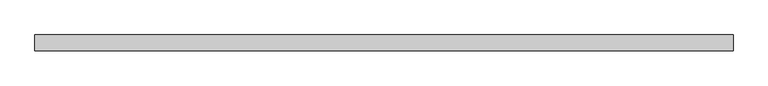
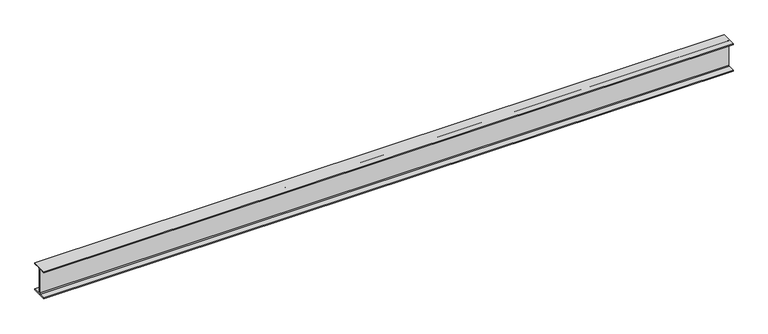
"""IFC4 building model written with IfcOpenShell, lengths in millimetres: beam geometry, Old_Steel Beam_H-KSD3502 : H_SB_ASB_H-390×300x10x16."""

import ifcopenshell
import ifcopenshell.guid

model = None  # the IFC model being written
_history = None  # IfcOwnerHistory: only IFC2X3 demands one
_inside = {}  # id of a spatial element -> (the spatial element, [elements in it])
_under = {}  # id of a project, library or spatial element -> (it, [spatial elements below it])
_declared = {}  # id of a project -> (the project, [libraries it declares])
_typed = {}  # id of a type object -> (the type object, [elements of that type])
_made_of = {}  # id of a material, layer set ... -> (it, [elements and type objects made of it])


def new_model(schema):
    """Start an empty IFC model of exactly this schema.

    Asked for "IFC4X3", IfcOpenShell would pick the latest addendum, in which some entities
    have other attributes; the version numbers below select the first issue.
    IFC2X3 requires an IfcOwnerHistory on every rooted entity: one is made here for all.
    """
    global model, _history
    if schema == "IFC4X3":
        model = ifcopenshell.file(schema_version=(4, 3, 0, 0))
    else:
        model = ifcopenshell.file(schema=schema)
    _inside.clear()
    _under.clear()
    _declared.clear()
    _typed.clear()
    _made_of.clear()
    _history = None
    if model.schema == "IFC2X3":
        org = make("IfcOrganization", Name="unknown")
        user = make(
            "IfcPersonAndOrganization",
            ThePerson=make("IfcPerson", FamilyName="unknown"),
            TheOrganization=org,
        )
        app = make(
            "IfcApplication",
            ApplicationDeveloper=org,
            Version="unknown",
            ApplicationFullName="unknown",
            ApplicationIdentifier="unknown",
        )
        _history = make(
            "IfcOwnerHistory",
            OwningUser=user,
            OwningApplication=app,
            ChangeAction="ADDED",
            CreationDate=0,
        )
    return model


def make(cls, **values):
    """One entity of the class cls with the attributes given. An attribute that is None is left unset."""
    return model.create_entity(
        cls, **{name: value for name, value in values.items() if value is not None}
    )


def rooted(cls, **values):
    """An entity with a GlobalId (a new one), such as an element, a storey or a relation."""
    return make(cls, GlobalId=ifcopenshell.guid.new(), OwnerHistory=_history, **values)


def si_unit(unit_type, name, prefix=None):
    """IfcSIUnit, for example si_unit("LENGTHUNIT", "METRE", prefix="MILLI")."""
    return make("IfcSIUnit", UnitType=unit_type, Prefix=prefix, Name=name)


def assignment(units):
    """IfcUnitAssignment: the units of a project."""
    return None if units is None else make("IfcUnitAssignment", Units=units)


def point(xyz):
    """IfcCartesianPoint."""
    return None if xyz is None else make("IfcCartesianPoint", Coordinates=xyz)


def direction(xyz):
    """IfcDirection."""
    return None if xyz is None else make("IfcDirection", DirectionRatios=xyz)


def frame(location, z_axis=None, x_axis=None):
    """IfcAxis2Placement3D, a coordinate frame: its origin and axes. An axis left out is left unset."""
    return make(
        "IfcAxis2Placement3D",
        Location=point(location),
        Axis=direction(z_axis),
        RefDirection=direction(x_axis),
    )


def frame_2d(location, x_axis=None):
    """IfcAxis2Placement2D, a coordinate frame in the plane: its origin and x axis."""
    return make(
        "IfcAxis2Placement2D", Location=point(location), RefDirection=direction(x_axis)
    )


def origin():
    """The frame at (0, 0, 0) with its axes left unset."""
    return frame((0.0, 0.0, 0.0))


def place(relative_to, where):
    """IfcLocalPlacement: puts the frame where relative to a parent placement (None: the world)."""
    return make(
        "IfcLocalPlacement", PlacementRelTo=relative_to, RelativePlacement=where
    )


def context(
    kind, dimensions, precision=None, world=None, true_north=None, identifier=None
):
    """IfcGeometricRepresentationContext, for example the 3D "Model" context."""
    return make(
        "IfcGeometricRepresentationContext",
        ContextIdentifier=identifier,
        ContextType=kind,
        CoordinateSpaceDimension=dimensions,
        Precision=precision,
        WorldCoordinateSystem=world,
        TrueNorth=true_north,
    )


def project(units=None, contexts=None):
    """IfcProject with its units and contexts."""
    return rooted(
        "IfcProject",
        Name="project",
        RepresentationContexts=contexts,
        UnitsInContext=assignment(units),
    )


def spatial(cls, under=None, at=None, **own):
    """A site, building, storey or space (cls), placed at a placement, below another one or the project."""
    s = rooted(cls, ObjectPlacement=at, **own)
    if under is not None:
        _under.setdefault(under.id(), (under, []))[1].append(s)
    return s


def polyline(points):
    """IfcPolyline through the points."""
    return make("IfcPolyline", Points=[point(p) for p in points])


def circle_curve(where, radius):
    """IfcCircle in the frame where."""
    return make("IfcCircle", Position=where, Radius=radius)


def trimmed(basis, trim1, trim2, sense, master):
    """IfcTrimmedCurve: the piece of a basis curve between two trims."""
    return make(
        "IfcTrimmedCurve",
        BasisCurve=basis,
        Trim1=trim1,
        Trim2=trim2,
        SenseAgreement=sense,
        MasterRepresentation=master,
    )


def segment(curve, same_sense, transition):
    """IfcCompositeCurveSegment."""
    return make(
        "IfcCompositeCurveSegment",
        Transition=transition,
        SameSense=same_sense,
        ParentCurve=curve,
    )


def composite_curve(segments, self_intersect=None):
    """IfcCompositeCurve: segments joined end to end."""
    return make("IfcCompositeCurve", Segments=segments, SelfIntersect=self_intersect)


def outline(outer, holes=None, kind="AREA"):
    """IfcArbitraryClosedProfileDef: a profile drawn as a closed curve; with holes, ...WithVoids."""
    if holes is None:
        return make("IfcArbitraryClosedProfileDef", ProfileType=kind, OuterCurve=outer)
    return make(
        "IfcArbitraryProfileDefWithVoids",
        ProfileType=kind,
        OuterCurve=outer,
        InnerCurves=holes,
    )


def extrude(swept, where, along, depth):
    """IfcExtrudedAreaSolid: the profile swept, set in the frame where, extruded along a direction by depth."""
    return make(
        "IfcExtrudedAreaSolid",
        SweptArea=swept,
        Position=where,
        ExtrudedDirection=direction(along),
        Depth=depth,
    )


def shape(context_of_items, identifier, shape_type, items):
    """IfcShapeRepresentation: the items that make up one representation, for example the "Body"."""
    return make(
        "IfcShapeRepresentation",
        ContextOfItems=context_of_items,
        RepresentationIdentifier=identifier,
        RepresentationType=shape_type,
        Items=items,
    )


def source(mapping_origin, context_of_items, identifier, shape_type, items):
    """IfcRepresentationMap: a shape defined once, which mapped items show again and again."""
    return make(
        "IfcRepresentationMap",
        MappingOrigin=mapping_origin,
        MappedRepresentation=shape(context_of_items, identifier, shape_type, items),
    )


def transform(
    local_origin,
    x_axis=None,
    y_axis=None,
    z_axis=None,
    scale=None,
    scale2=None,
    scale3=None,
    uniform=True,
):
    """IfcCartesianTransformationOperator3D, or its non-uniform kind. x_axis, y_axis, z_axis: its Axis1, 2, 3."""
    if uniform:
        return make(
            "IfcCartesianTransformationOperator3D",
            Axis1=direction(x_axis),
            Axis2=direction(y_axis),
            LocalOrigin=point(local_origin),
            Scale=scale,
            Axis3=direction(z_axis),
        )
    return make(
        "IfcCartesianTransformationOperator3DnonUniform",
        Axis1=direction(x_axis),
        Axis2=direction(y_axis),
        LocalOrigin=point(local_origin),
        Scale=scale,
        Axis3=direction(z_axis),
        Scale2=scale2,
        Scale3=scale3,
    )


def mapped(mapping_source, mapping_target):
    """IfcMappedItem: shows the shape of a source again, moved by a transform."""
    return make(
        "IfcMappedItem", MappingSource=mapping_source, MappingTarget=mapping_target
    )


def made_of(thing, what):
    """Note that an element or type object is made of a material, layer set ...; save() writes the relation."""
    if what is not None:
        _made_of.setdefault(what.id(), (what, []))[1].append(thing)
    return thing


def element(
    cls,
    number,
    at=None,
    inside=None,
    cuts=None,
    type_object=None,
    material=None,
    context=None,
    identifier="Body",
    shape_type=None,
    held_by="IfcProductDefinitionShape",
    body=None,
    shapes=None,
    **own,
):
    """One element of the class cls, such as IfcWall. Its Tag is "e" and its number.

    at: its placement. inside: the storey or other place that contains it. cuts: it is an
    opening in that element (IfcRelVoidsElement). A single representation is given by context,
    identifier, shape_type and body (its items); several are given by shapes. held_by: the class
    of the entity that holds the representations. save() writes the other relations.
    """
    e = rooted(cls, Tag="e%d" % number, ObjectPlacement=at, **own)
    if body is not None:
        shapes = [shape(context, identifier, shape_type, body)]
    if shapes is not None:
        e.Representation = make(held_by, Representations=shapes)
    if inside is not None:
        _inside.setdefault(inside.id(), (inside, []))[1].append(e)
    if cuts is not None:
        rooted(
            "IfcRelVoidsElement", RelatingBuildingElement=cuts, RelatedOpeningElement=e
        )
    if type_object is not None:
        _typed.setdefault(type_object.id(), (type_object, []))[1].append(e)
    return made_of(e, material)


def aggregate(whole, parts):
    """IfcRelAggregates: a whole, such as a stair, and the parts it consists of."""
    return rooted("IfcRelAggregates", RelatingObject=whole, RelatedObjects=parts)


def save(model, path):
    """Write the relations noted so far, then the file.

    IfcRelAggregates (storeys below a building ...), IfcRelContainedInSpatialStructure (elements
    in a storey), IfcRelDefinesByType, IfcRelAssociatesMaterial and IfcRelDeclares: one each for
    every whole, place, type object, material and project.
    """
    for whole, parts in _under.values():
        aggregate(whole, parts)
    for where, things in _inside.values():
        rooted(
            "IfcRelContainedInSpatialStructure",
            RelatedElements=things,
            RelatingStructure=where,
        )
    for kind, things in _typed.values():
        rooted("IfcRelDefinesByType", RelatedObjects=things, RelatingType=kind)
    for what, things in _made_of.values():
        rooted("IfcRelAssociatesMaterial", RelatedObjects=things, RelatingMaterial=what)
    for by, libraries in _declared.values():
        rooted("IfcRelDeclares", RelatingContext=by, RelatedDefinitions=libraries)
    model.write(path)


def beam_ac0c7c79(model_context):
    return source(origin(), model_context, "Body", "SweptSolid", [
        extrude(outline(composite_curve([segment(polyline([(82.5, -141.5), (82.5, -151.7), (-82.5, -151.7), (-82.5, -141.5), (-11.9, -141.5)]), True, "CONTINUOUS"), segment(trimmed(circle_curve(frame_2d((-11.9, -132.6)), 8.9), [point((-11.9, -141.5))], [point((-3.0, -132.6))], True, "CARTESIAN"), True, "CONTINUOUS"), segment(polyline([(-3.0, -132.6), (-3.0, 132.6)]), True, "CONTINUOUS"), segment(trimmed(circle_curve(frame_2d((-11.9, 132.6)), 8.9), [point((-3.0, 132.6))], [point((-11.9, 141.5))], True, "CARTESIAN"), True, "CONTINUOUS"), segment(polyline([(-11.9, 141.5), (-82.5, 141.5), (-82.5, 151.7), (82.5, 151.7), (82.5, 141.5), (11.9, 141.5)]), True, "CONTINUOUS"), segment(trimmed(circle_curve(frame_2d((11.9, 132.6)), 8.9), [point((11.9, 141.5))], [point((3.0, 132.6))], True, "CARTESIAN"), True, "CONTINUOUS"), segment(polyline([(3.0, 132.6), (3.0, -132.6)]), True, "CONTINUOUS"), segment(trimmed(circle_curve(frame_2d((11.9, -132.6)), 8.9), [point((3.0, -132.6))], [point((11.9, -141.5))], True, "CARTESIAN"), True, "CONTINUOUS"), segment(polyline([(11.9, -141.5), (82.5, -141.5)]), True, "CONTINUOUS")], self_intersect=False)), frame((-3764.034879, 0.0, 0.0), z_axis=(1.0, 0.0, 0.0), x_axis=(0.0, 1.0, 0.0)), (0.0, 0.0, 1.0), 7251.3348784),
    ])


if __name__ == "__main__":
    model = new_model("IFC4")
    model_context = context("Model", 3, world=origin())
    ifc_project = project(units=[si_unit("LENGTHUNIT", "METRE", prefix="MILLI")], contexts=[model_context])
    site = spatial("IfcSite", under=ifc_project)
    building = spatial("IfcBuilding", under=site)
    placement = place(None, origin())
    beam_shape = beam_ac0c7c79(model_context)
    element("IfcBeam", 1, ObjectType="Old_Steel Beam_H-KSD3502 : H_SB_ASB_H-390×300x10x16", at=placement, inside=building, context=model_context, shape_type="MappedRepresentation", body=[
        mapped(beam_shape, transform((0.0, 0.0, 0.0), x_axis=(1.0, 0.0, 0.0), y_axis=(0.0, 1.0, 0.0), z_axis=(0.0, 0.0, 1.0))),
    ])
    save(model, "model.ifc")

# Revit data of these elements
# Type "Old_Steel Beam_H-KSD3502 : H_SB_ASB_H-390×300x10x16"
#   Width = 30.0 cm
#   Web Thickness = 1.0 cm
#   Web Fillet = 2.2 cm
#   Warping Constant = 2517770.0 cm⁶
#   Torsional Moment of Inertia = 94.3867 cm⁴
#   Torsional Modulus = 1.0 cm³
#   Section Area = 136.0 cm²
#   Plastic Modulus weak axis = 733.0 cm³
#   Plastic Modulus strong axis = 2190.0 cm³
#   Perimeter = 1.92 m²/m
#   Nominal Weight = 107.00 kgf/m
#   Moment of Inertia weak axis = 7210.00 cm⁴
#   Moment of Inertia strong axis = 38700.00 cm⁴
#   Height = 39.0 cm
#   Flange Thickness = 1.6 cm
#   Elastic Modulus weak axis = 481.0 cm³
#   Elastic Modulus strong axis = 1980.0 cm³
#   Centroid Vertical = 19.5 cm
#   Centroid Horizontal = 15.0 cm
#   Length [instance default] = 1.5240 m
#   Structural Material [instance default] = Steel, 45-345
#   Assembly Code = ""
# Element 1 (IfcBeam, "Old_Steel Beam_H-KSD3502 : H_SB_ASB_H-390×300x10x16")
#   Structural Material = none
# Materials
#   "Steel, 45-345": class "Metal", colour RGB 189 187 185, transparency 0, Description = "Steel 345 MPa", Cost = 0
